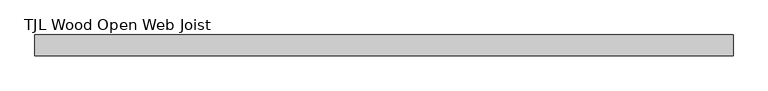
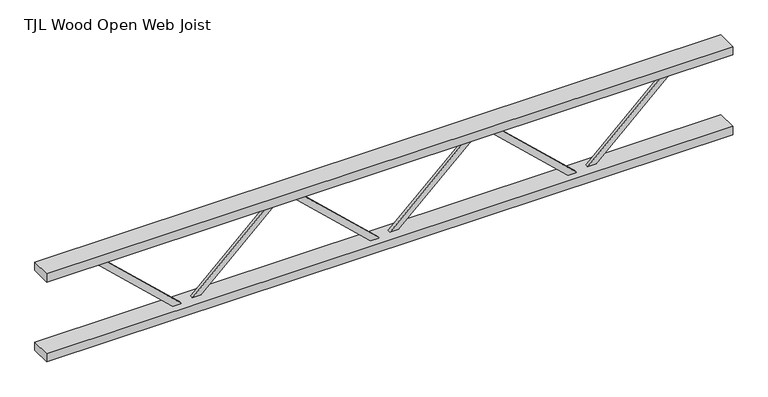
"""IFC4 building model written with IfcOpenShell, lengths in millimetres: beam geometry, TJL Wood Open Web Joist."""

from ifc_helpers import new_model, si_unit, frame, origin, place, context, project, spatial, polyline, outline, extrude, source, transform, mapped, element, save


def tjl_wood_open_web_joist_00f6e9cf(model_context):
    return source(origin(), model_context, "Body", "SweptSolid", [
        extrude(outline(polyline([(171.45, 431.5354167), (196.85, 431.5354167), (196.85, 413.8186573), (-171.45, 20.3832406), (-171.45, -25.4), (-196.85, -25.4), (-196.85, 30.4167594), (171.45, 423.852176), (171.45, 431.5354167)])), frame((0.0, 0.0, 0.0), z_axis=(0.0, 1.0, 0.0), x_axis=(0.0, 0.0, 1.0)), (0.0, 0.0, 1.0), 12.7),
        extrude(outline(polyline([(196.85, -431.5354167), (171.45, -431.5354167), (171.45, -423.852176), (-196.85, -30.4167594), (-196.85, 25.4), (-171.45, 25.4), (-171.45, -20.3832406), (196.85, -413.8186573), (196.85, -431.5354167)])), frame((0.0, -12.7, 0.0), z_axis=(0.0, 1.0, 0.0), x_axis=(0.0, 0.0, 1.0)), (0.0, 0.0, 1.0), 12.7),
        extrude(outline(polyline([(171.45, 1294.60625), (196.85, 1294.60625), (196.85, 1276.8894906), (-171.45, 883.454074), (-171.45, 837.6708333), (-196.85, 837.6708333), (-196.85, 893.4875927), (171.45, 1286.9230094), (171.45, 1294.60625)])), frame((0.0, 0.0, 0.0), z_axis=(0.0, 1.0, 0.0), x_axis=(0.0, 0.0, 1.0)), (0.0, 0.0, 1.0), 12.7),
        extrude(outline(polyline([(196.85, 431.5354167), (171.45, 431.5354167), (171.45, 439.2186573), (-196.85, 832.654074), (-196.85, 888.4708333), (-171.45, 888.4708333), (-171.45, 842.6875927), (196.85, 449.252176), (196.85, 431.5354167)])), frame((0.0, -12.7, 0.0), z_axis=(0.0, 1.0, 0.0), x_axis=(0.0, 0.0, 1.0)), (0.0, 0.0, 1.0), 12.7),
        extrude(outline(polyline([(171.45, -431.5354167), (196.85, -431.5354167), (196.85, -449.252176), (-171.45, -842.6875927), (-171.45, -888.4708333), (-196.85, -888.4708333), (-196.85, -832.654074), (171.45, -439.2186573), (171.45, -431.5354167)])), frame((0.0, 0.0, 0.0), z_axis=(0.0, 1.0, 0.0), x_axis=(0.0, 0.0, 1.0)), (0.0, 0.0, 1.0), 12.7),
        extrude(outline(polyline([(196.85, -1294.60625), (171.45, -1294.60625), (171.45, -1286.9230094), (-196.85, -893.4875927), (-196.85, -837.6708333), (-171.45, -837.6708333), (-171.45, -883.454074), (196.85, -1276.8894906), (196.85, -1294.60625)])), frame((0.0, -12.7, 0.0), z_axis=(0.0, 1.0, 0.0), x_axis=(0.0, 0.0, 1.0)), (0.0, 0.0, 1.0), 12.7),
        extrude(outline(polyline([(1497.80625, 44.45), (1497.80625, -44.45), (-1497.80625, -44.45), (-1497.80625, 44.45), (1497.80625, 44.45)])), frame((0.0, 0.0, 165.1), z_axis=(0.0, 0.0, 1.0), x_axis=(1.0, 0.0, 0.0)), (0.0, 0.0, 1.0), 38.1),
        extrude(outline(polyline([(1497.80625, 44.45), (1497.80625, -44.45), (-1497.80625, -44.45), (-1497.80625, 44.45), (1497.80625, 44.45)])), frame((0.0, 0.0, -203.2), z_axis=(0.0, 0.0, 1.0), x_axis=(1.0, 0.0, 0.0)), (0.0, 0.0, 1.0), 38.1),
    ])


if __name__ == "__main__":
    model = new_model("IFC4")
    model_context = context("Model", 3, world=origin())
    ifc_project = project(units=[si_unit("LENGTHUNIT", "METRE", prefix="MILLI")], contexts=[model_context])
    site = spatial("IfcSite", under=ifc_project)
    building = spatial("IfcBuilding", under=site)
    placement = place(None, origin())
    tjl_wood_open_web_joist_shape = tjl_wood_open_web_joist_00f6e9cf(model_context)
    element("IfcBeam", 1, ObjectType="TJL Wood Open Web Joist : 16\" PREENGINEERED FLOOR TRUSS", at=placement, inside=building, context=model_context, shape_type="MappedRepresentation", body=[
        mapped(tjl_wood_open_web_joist_shape, transform((0.0, 0.0, 0.0), x_axis=(1.0, 0.0, 0.0), y_axis=(0.0, 1.0, 0.0), z_axis=(0.0, 0.0, 1.0))),
    ])
    save(model, "model.ifc")

# Revit data of these elements
# Type "TJL Wood Open Web Joist : 16\" PREENGINEERED FLOOR TRUSS"
#   Web Thickness = 0' - 1"
#   Web Leg = 0' - 1"
#   Start Offset [instance default] = 0' - 0"
#   Top Chord Start Extension [instance default] = 0' - 0"
#   PanelArrayLength [instance default] = 22' - 8"
#   Depth = 1' - 4"
#   PanelWidth [instance default] = 2' - 6.22222"
#   Offset Length 2 [instance default] = 0' - 8"
#   Offset Length 1 [instance default] = 0' - 8"
#   End Panel [instance default] = 0' - 8"
#   End Offset [instance default] = 0' - 0"
#   Top Chord End Extension [instance default] = 0' - 0"
#   Chord Width = 0' - 3 1/2"
#   Chord Depth = 0' - 1 1/2"
#   Bottom Chord Start Extension [instance default] = 0' - 0"
#   Bottom Chord End Extension [instance default] = 0' - 0"
#   Length [instance default] = 24' - 0"
#   PanelArrayNum [instance default] = 9
#   Web Rendering Material = none
#   Structural Material = none
#   Assembly Code = ""
# Element 1 (IfcBeam, "TJL Wood Open Web Joist : 16\" PREENGINEERED FLOOR TRUSS")
#   PanelArrayLength = 8' - 5 15/16"
#   PanelWidth = 2' - 9.97917"
#   PanelArrayNum = 3
